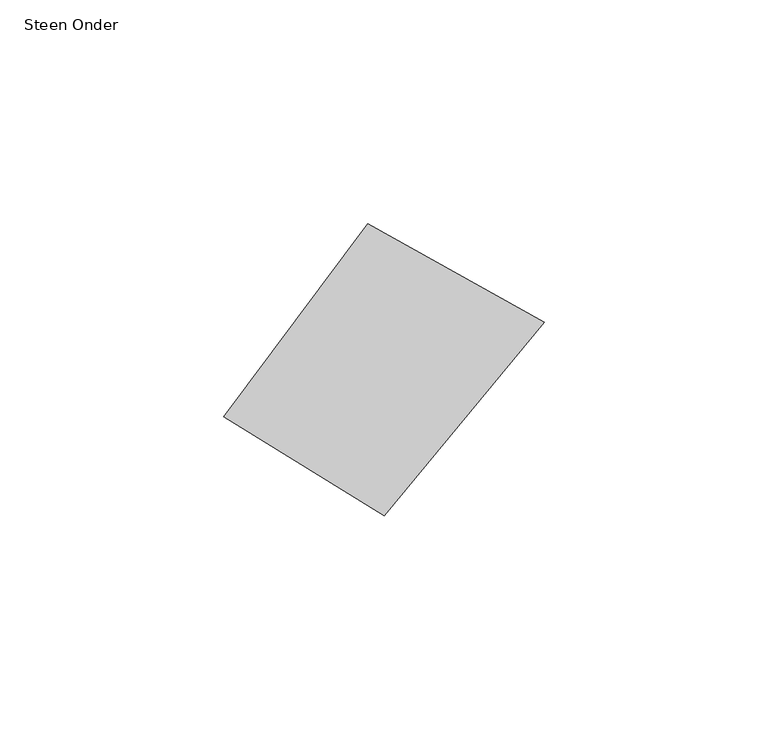
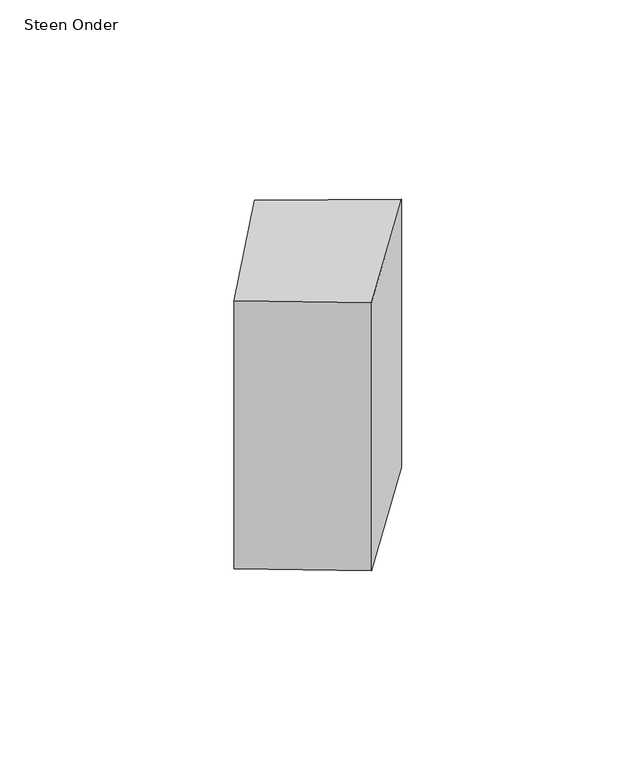
"""IFC4 building model written with IfcOpenShell, lengths in millimetres: proxy geometry, 00_GMA_steen_versie_4 : Steen Onder."""

from ifc_helpers import new_model, si_unit, frame, origin, place, context, project, spatial, polyline, outline, extrude, source, transform, mapped, element, save


def steen_onder_2ab03e8d(model_context):
    return source(origin(), model_context, "Body", "SweptSolid", [
        extrude(outline(polyline([(120.1156098, 54.8222151), (84.4304447, 11.5711708), (48.6108657, 33.657145), (80.7305785, 76.736296), (120.1156098, 54.8222151)])), frame((0.0, 0.0, -100.0), z_axis=(0.0, 0.0, 1.0), x_axis=(1.0, 0.0, 0.0)), (0.0, 0.0, 1.0), 100.0),
    ])


if __name__ == "__main__":
    model = new_model("IFC4")
    model_context = context("Model", 3, world=origin())
    ifc_project = project(units=[si_unit("LENGTHUNIT", "METRE", prefix="MILLI")], contexts=[model_context])
    site = spatial("IfcSite", under=ifc_project)
    building = spatial("IfcBuilding", under=site)
    placement = place(None, origin())
    steen_onder_shape = steen_onder_2ab03e8d(model_context)
    element("IfcBuildingElementProxy", 1, Name="00_GMA_steen_versie_4 : Steen Onder", ObjectType="00_GMA_steen_versie_4 : Steen Onder", at=placement, inside=building, context=model_context, shape_type="MappedRepresentation", body=[
        mapped(steen_onder_shape, transform((0.0, 0.0, 0.0), x_axis=(1.0, 0.0, 0.0), y_axis=(0.0, 1.0, 0.0), z_axis=(0.0, 0.0, 1.0))),
    ])
    save(model, "model.ifc")

# Revit data of these elements
# Type "00_GMA_steen_versie_4 : Steen Onder"
#   StootVoegHalfBoven [instance default] = 5 mm
#   StootVoegHalf [instance default] = 5 mm
#   StootVoegBreedteOnder = 10 mm
#   StootVoegBreedteBoven = 10 mm
#   Steendikte = 100 mm
#   LintVoegOnderHalf = 0 mm
#   LintVoegOnder = 0 mm
#   LintVoegBovenHalf = 5 mm
#   LintVoegBoven = 10 mm
#   materiaal = none
#   MateriaalVoeg = none
#   Default Elevation = 0
